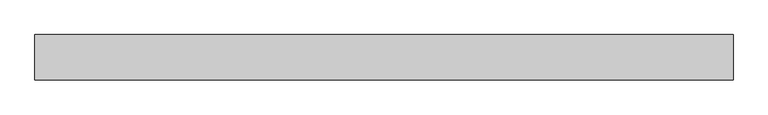
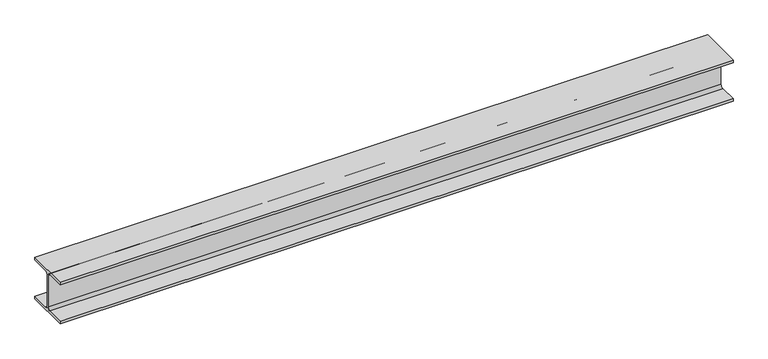
"""IFC4 building model written with IfcOpenShell, lengths in millimetres: beam geometry, 0912_Steel Framing_H-KSD3502 : H_SB_ASB_H-200x200x8x12."""

from ifc_helpers import new_model, si_unit, point, frame, frame_2d, origin, place, context, project, spatial, polyline, circle_curve, trimmed, segment, composite_curve, outline, extrude, source, transform, mapped, element, save


def beam_b47cc47b(model_context):
    return source(origin(), model_context, "Body", "SweptSolid", [
        extrude(outline(composite_curve([segment(polyline([(100.0, -88.0), (100.0, -100.0), (-100.0, -100.0), (-100.0, -88.0), (-17.0, -88.0)]), True, "CONTINUOUS"), segment(trimmed(circle_curve(frame_2d((-17.0, -75.0)), 13.0), [point((-17.0, -88.0))], [point((-4.0, -75.0))], True, "CARTESIAN"), True, "CONTINUOUS"), segment(polyline([(-4.0, -75.0), (-4.0, 75.0)]), True, "CONTINUOUS"), segment(trimmed(circle_curve(frame_2d((-17.0, 75.0)), 13.0), [point((-4.0, 75.0))], [point((-17.0, 88.0))], True, "CARTESIAN"), True, "CONTINUOUS"), segment(polyline([(-17.0, 88.0), (-100.0, 88.0), (-100.0, 100.0), (100.0, 100.0), (100.0, 88.0), (17.0, 88.0)]), True, "CONTINUOUS"), segment(trimmed(circle_curve(frame_2d((17.0, 75.0)), 13.0), [point((17.0, 88.0))], [point((4.0, 75.0))], True, "CARTESIAN"), True, "CONTINUOUS"), segment(polyline([(4.0, 75.0), (4.0, -75.0)]), True, "CONTINUOUS"), segment(trimmed(circle_curve(frame_2d((17.0, -75.0)), 13.0), [point((4.0, -75.0))], [point((17.0, -88.0))], True, "CARTESIAN"), True, "CONTINUOUS"), segment(polyline([(17.0, -88.0), (100.0, -88.0)]), True, "CONTINUOUS")], self_intersect=False)), frame((-1348.7293089, 0.0, 0.0), z_axis=(1.0, 0.0, 0.0), x_axis=(0.0, 1.0, 0.0)), (0.0, 0.0, 1.0), 3072.1818503),
    ])


if __name__ == "__main__":
    model = new_model("IFC4")
    model_context = context("Model", 3, world=origin())
    ifc_project = project(units=[si_unit("LENGTHUNIT", "METRE", prefix="MILLI")], contexts=[model_context])
    site = spatial("IfcSite", under=ifc_project)
    building = spatial("IfcBuilding", under=site)
    placement = place(None, origin())
    beam_shape = beam_b47cc47b(model_context)
    element("IfcBeam", 1, ObjectType="0912_Steel Framing_H-KSD3502 : H_SB_ASB_H-200x200x8x12", at=placement, inside=building, context=model_context, shape_type="MappedRepresentation", body=[
        mapped(beam_shape, transform((0.0, 0.0, 0.0), x_axis=(1.0, 0.0, 0.0), y_axis=(0.0, 1.0, 0.0), z_axis=(0.0, 0.0, 1.0))),
    ])
    save(model, "model.ifc")

# Revit data of these elements
# Type "0912_Steel Framing_H-KSD3502 : H_SB_ASB_H-200x200x8x12"
#   H_WM Code_1 = "S01AA002-00001 | Main Steel Structure Fabrication Work | Shelter/Building | Medium Steel - Standard (90KG/M>Weight≥30KG/M) | Material: (   )"
#   H_WM Code_2 = "S03AA028-00001 | Main Steel Structure Erection Work | Shelter/Building | Medium Steel (90KG/M>Weight≥30KG/M) | Material: (   )"
#   H_WM Code_3 = "S01AA010-00001 | Main Steel Structure Fabrication Work | Shelter/Building | Steel Painting/Coating | for Non-Fireproofed Steel Surface, Surface Preparation, Primer, Second & Final Coat | Material: (   )"
#   H_Q'ty Cal Type Tag = "SB-Q2"
#   Width = 20.0 cm
#   Web Thickness = 0.8 cm
#   Web Fillet = 1.3 cm
#   Warping Constant = 141000.0 cm⁶
#   W = 0
#   Torsional Moment of Inertia = 26.2485 cm⁴
#   Section Area = 63.53 cm²
#   Plastic Modulus weak axis = 244.0 cm³
#   Plastic Modulus strong axis = 525.0 cm³
#   Perimeter = 1.16 m²/m
#   Nominal Weight = 49.90 kgf/m
#   Moment of Inertia weak axis = 1600.00 cm⁴
#   Moment of Inertia strong axis = 4720.00 cm⁴
#   Height = 20.0 cm
#   Flange Thickness = 1.2 cm
#   Elastic Modulus weak axis = 160.0 cm³
#   Elastic Modulus strong axis = 472.0 cm³
#   Centroid Vertical = 10.0 cm
#   Centroid Horizontal = 10.0 cm
#   Ix = 47200000
#   Length [instance default] = 1.5240 m
#   Zx = 525000
#   b = 0.2000 m
#   h = 0.2000 m
#   r = 0.0130 m
#   s = 0.0080 m
#   t = 0.0120 m
#   A = 0.006353 m²
#   Structural Material [instance default] = Steel, 45-345
#   Assembly Code = ""
# Element 1 (IfcBeam, "0912_Steel Framing_H-KSD3502 : H_SB_ASB_H-200x200x8x12")
#   Structural Material = none
# Materials
#   "Steel, 45-345": class "Metal", colour RGB 189 187 185, transparency 0, Description = "Steel 345 MPa", Cost = 0
